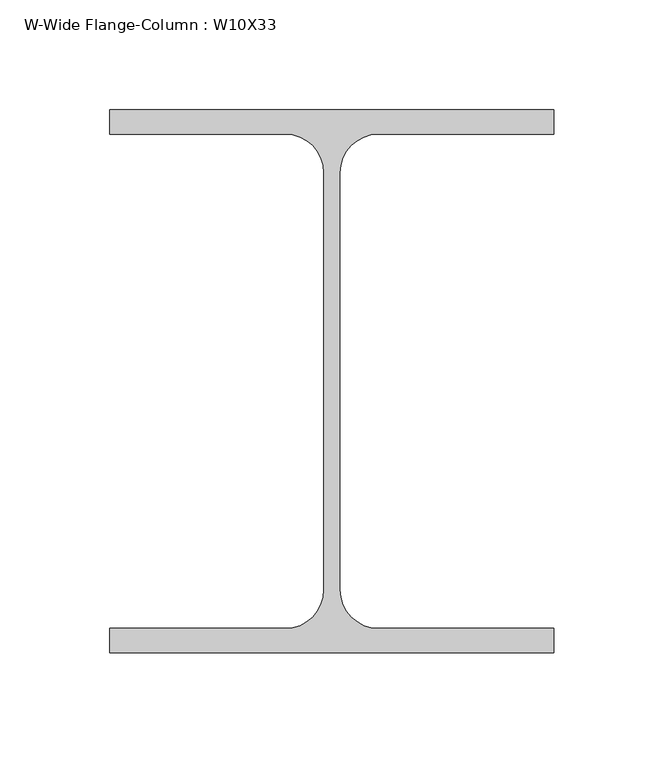
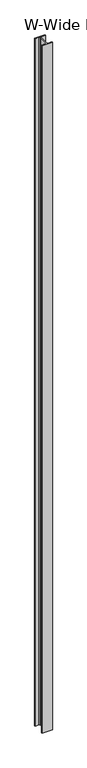
"""IFC4 building model written with IfcOpenShell, lengths in millimetres: column geometry, W-Wide Flange-Column : W10X33."""

from ifc_helpers import new_model, si_unit, point, frame, frame_2d, origin, place, context, project, spatial, polyline, circle_curve, trimmed, segment, composite_curve, outline, extrude, source, transform, mapped, element, save


def w_wide_flange_column_w10x33_b6efe3a9(model_context):
    return source(origin(), model_context, "Body", "SweptSolid", [
        extrude(outline(composite_curve([segment(polyline([(101.092, 123.571), (101.092, 112.522), (21.209, 112.522)]), True, "CONTINUOUS"), segment(trimmed(circle_curve(frame_2d((21.209, 94.996)), 17.526), [point((21.209, 112.522))], [point((3.683, 94.996))], True, "CARTESIAN"), True, "CONTINUOUS"), segment(polyline([(3.683, 94.996), (3.683, -94.996)]), True, "CONTINUOUS"), segment(trimmed(circle_curve(frame_2d((21.209, -94.996)), 17.526), [point((3.683, -94.996))], [point((21.209, -112.522))], True, "CARTESIAN"), True, "CONTINUOUS"), segment(polyline([(21.209, -112.522), (101.092, -112.522), (101.092, -123.571), (-101.092, -123.571), (-101.092, -112.522), (-21.209, -112.522)]), True, "CONTINUOUS"), segment(trimmed(circle_curve(frame_2d((-21.209, -94.996)), 17.526), [point((-21.209, -112.522))], [point((-3.683, -94.996))], True, "CARTESIAN"), True, "CONTINUOUS"), segment(polyline([(-3.683, -94.996), (-3.683, 94.996)]), True, "CONTINUOUS"), segment(trimmed(circle_curve(frame_2d((-21.209, 94.996)), 17.526), [point((-3.683, 94.996))], [point((-21.209, 112.522))], True, "CARTESIAN"), True, "CONTINUOUS"), segment(polyline([(-21.209, 112.522), (-101.092, 112.522), (-101.092, 123.571), (101.092, 123.571)]), True, "CONTINUOUS")], self_intersect=False)), frame((0.0, 0.0, 13379.45), z_axis=(0.0, 0.0, 1.0), x_axis=(1.0, 0.0, 0.0)), (0.0, 0.0, 1.0), 14204.95),
    ])


if __name__ == "__main__":
    model = new_model("IFC4")
    model_context = context("Model", 3, world=origin())
    ifc_project = project(units=[si_unit("LENGTHUNIT", "METRE", prefix="MILLI")], contexts=[model_context])
    site = spatial("IfcSite", under=ifc_project)
    building = spatial("IfcBuilding", under=site)
    placement = place(None, origin())
    w_wide_flange_column_w10x33_shape = w_wide_flange_column_w10x33_b6efe3a9(model_context)
    element("IfcColumn", 1, ObjectType="W-Wide Flange-Column : W10X33", at=placement, inside=building, context=model_context, shape_type="MappedRepresentation", body=[
        mapped(w_wide_flange_column_w10x33_shape, transform((0.0, 0.0, 0.0), x_axis=(1.0, 0.0, 0.0), y_axis=(0.0, 1.0, 0.0), z_axis=(0.0, 0.0, 1.0))),
    ])
    save(model, "model.ifc")

# Revit data of these elements
# Type "W-Wide Flange-Column : W10X33"
#   Assembly Code = "B10"
#   W = 33
#   bf = 0' - 7.96"
#   d = 0' - 9.73"
#   k = 0' - 1 1/8"
#   kr = 0' - 0.69"
#   tf = 0' - 0.435"
#   tw = 0' - 0.29"
#   A = 0.0674306 SF
#   Structural Material [instance default] = Steel ASTM A992
# Element 1 (IfcColumn, "W-Wide Flange-Column : W10X33")
#   Materials on its faces: "Steel ASTM A992"
# Materials
#   "Steel ASTM A992": class "Metal", colour RGB 199 199 199, transparency 0, Description = "Structural steel 50ksi", Cost = 0
